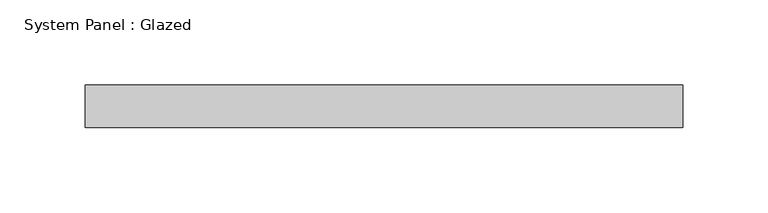
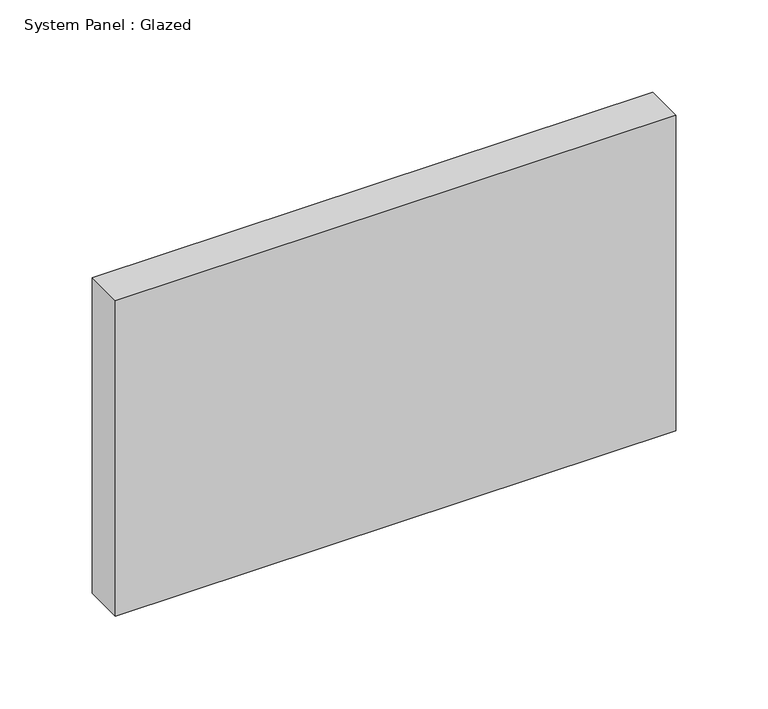
"""IFC4 building model written with IfcOpenShell, lengths in millimetres: plate geometry, System Panel : Glazed."""

from ifc_helpers import new_model, si_unit, origin, origin_with_axes, place, context, project, spatial, polyline, outline, extrude, source, transform, mapped, element, save


def system_panel_glazed_e40b210f(model_context):
    return source(origin(), model_context, "Body", "SweptSolid", [
        extrude(outline(polyline([(175.0, 24.5), (-175.0, 24.5), (-175.0, 49.5), (175.0, 49.5), (175.0, 24.5)])), origin_with_axes(), (0.0, 0.0, 1.0), 208.3333333),
    ])


if __name__ == "__main__":
    model = new_model("IFC4")
    model_context = context("Model", 3, world=origin())
    ifc_project = project(units=[si_unit("LENGTHUNIT", "METRE", prefix="MILLI")], contexts=[model_context])
    site = spatial("IfcSite", under=ifc_project)
    building = spatial("IfcBuilding", under=site)
    placement = place(None, origin())
    system_panel_glazed_shape = system_panel_glazed_e40b210f(model_context)
    element("IfcPlate", 1, ObjectType="System Panel : Glazed", at=placement, inside=building, context=model_context, shape_type="MappedRepresentation", body=[
        mapped(system_panel_glazed_shape, transform((0.0, 0.0, 0.0), x_axis=(1.0, 0.0, 0.0), y_axis=(0.0, 1.0, 0.0), z_axis=(0.0, 0.0, 1.0))),
    ])
    save(model, "model.ifc")

# Revit data of these elements
# Element 1 (IfcPlate, "System Panel : Glazed")
#   Materials on its faces: "Glass"
# Materials
#   "Glass": class "Glass", colour RGB 218 227 224, transparency 0.85, Description = "Soda Lime Glass", Cost = 0
